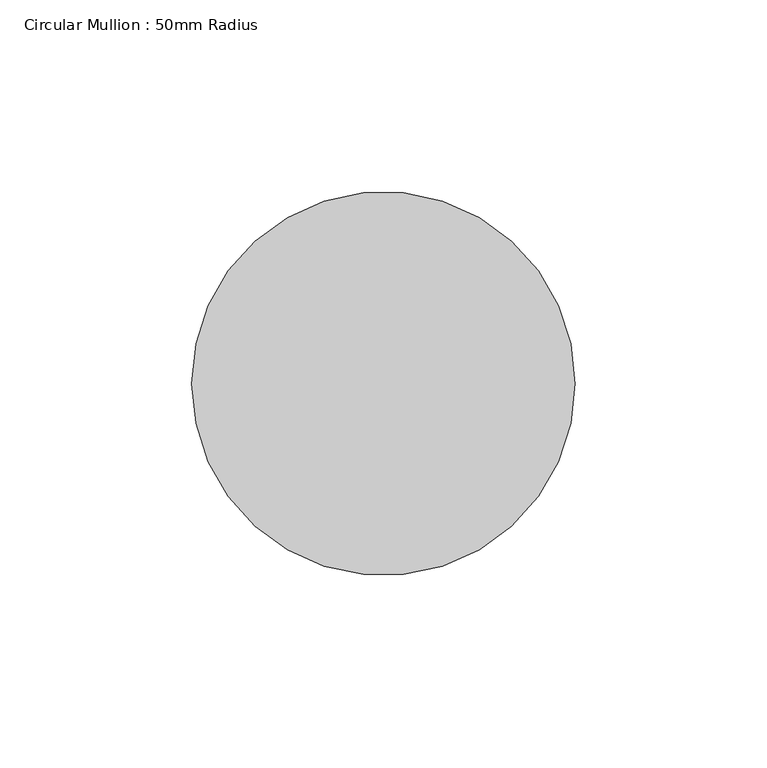
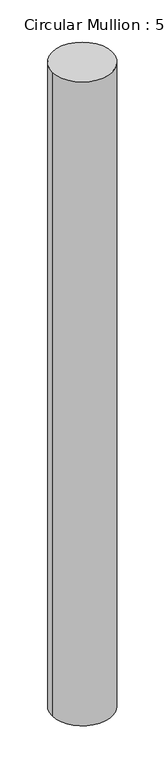
"""IFC4 building model written with IfcOpenShell, lengths in millimetres: member geometry, Circular Mullion : 50mm Radius."""

from ifc_helpers import new_model, si_unit, point, frame, origin, origin_2d, place, context, project, spatial, circle_curve, trimmed, segment, composite_curve, outline, extrude, source, transform, mapped, element, save


def circular_mullion_50mm_radius_978f2ed6(model_context):
    return source(origin(), model_context, "Body", "SweptSolid", [
        extrude(outline(composite_curve([segment(trimmed(circle_curve(origin_2d(), 50.0), [point((50.0, 0.0))], [point((-50.0, 0.0))], False, "CARTESIAN"), True, "CONTINUOUS"), segment(trimmed(circle_curve(origin_2d(), 50.0), [point((-50.0, 0.0))], [point((50.0, 0.0))], False, "CARTESIAN"), True, "CONTINUOUS")], self_intersect=False)), frame((0.0, 0.0, -1133.8994211), z_axis=(0.0, 0.0, 1.0), x_axis=(1.0, 0.0, 0.0)), (0.0, 0.0, 1.0), 1133.8994211),
    ])


if __name__ == "__main__":
    model = new_model("IFC4")
    model_context = context("Model", 3, world=origin())
    ifc_project = project(units=[si_unit("LENGTHUNIT", "METRE", prefix="MILLI")], contexts=[model_context])
    site = spatial("IfcSite", under=ifc_project)
    building = spatial("IfcBuilding", under=site)
    placement = place(None, origin())
    circular_mullion_50mm_radius_shape = circular_mullion_50mm_radius_978f2ed6(model_context)
    element("IfcMember", 1, ObjectType="Circular Mullion : 50mm Radius", at=placement, inside=building, context=model_context, shape_type="MappedRepresentation", body=[
        mapped(circular_mullion_50mm_radius_shape, transform((0.0, 0.0, 0.0), x_axis=(1.0, 0.0, 0.0), y_axis=(0.0, 1.0, 0.0), z_axis=(0.0, 0.0, 1.0))),
    ])
    save(model, "model.ifc")

# Revit data of these elements
# Type "Circular Mullion : 50mm Radius"
#   built-in parameter 1007350 = 0.164042 (stored number, unit not read)
# Element 1 (IfcMember, "Circular Mullion : 50mm Radius")
#   Materials on its faces: "Aluminium"
# Materials
#   "Aluminium": class "Metal", colour RGB 247 247 247, transparency 0, Description = "Aluminium 6061", Cost = 0
